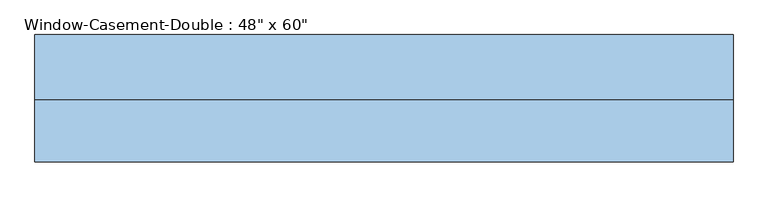
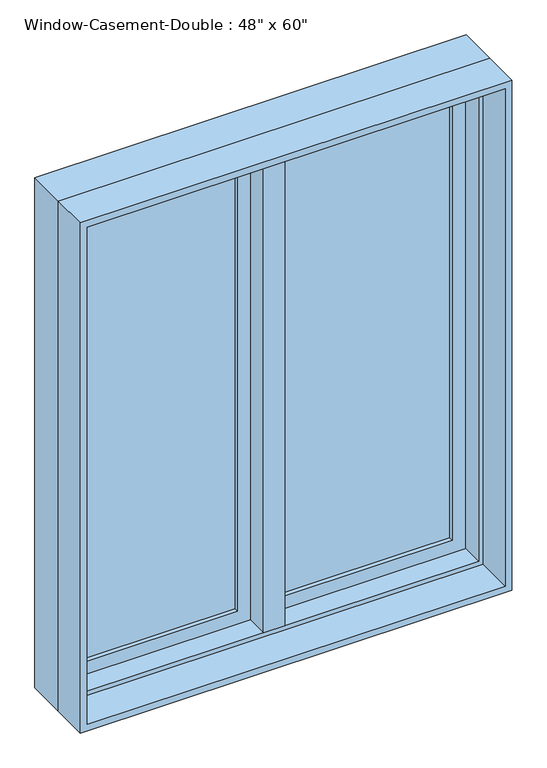
"""IFC4 building model written with IfcOpenShell, lengths in millimetres: window geometry."""

from ifc_helpers import new_model, si_unit, frame, origin, place, context, project, spatial, polyline, outline, extrude, faceted_brep, source, transform, mapped, element, save


def window_78633f8a(model_context):
    return source(origin(), model_context, "Body", "SolidModel", [
        faceted_brep([(9.525, 120.65, 2425.7), (-9.525, 120.65, 2425.7), (-9.525, 69.85, 2425.7), (9.525, 69.85, 2425.7), (9.525, 120.65, 927.1), (9.525, 69.85, 927.1), (-9.525, 69.85, 927.1), (-9.525, 120.65, 927.1), (-9.525, 69.85, 946.15), (-9.525, 69.85, 2406.65), (-30.1625, 69.85, 946.15), (-30.1625, 69.85, 2406.65), (-30.1625, 6.35, 946.15), (-30.1625, 6.35, 2406.65), (30.1625, 6.35, 946.15), (30.1625, 6.35, 2406.65), (30.1625, 69.85, 946.15), (30.1625, 69.85, 2406.65), (9.525, 69.85, 946.15), (9.525, 69.85, 2406.65)], [[[0, 1, 2, 3]], [[4, 5, 6, 7]], [[1, 0, 4, 7]], [[2, 1, 7, 6, 8, 9]], [[9, 8, 10, 11]], [[11, 10, 12, 13]], [[13, 12, 14, 15]], [[15, 14, 16, 17]], [[17, 16, 18, 19]], [[0, 3, 19, 18, 5, 4]], [[18, 8, 6, 5]], [[9, 19, 3, 2]], [[8, 18, 16, 14, 12, 10]], [[19, 9, 11, 13, 15, 17]]]),
        extrude(outline(polyline([(-66.675, 101.6), (-66.675, 95.25), (-539.75, 95.25), (-539.75, 101.6), (-66.675, 101.6)])), frame((0.0, 0.0, 984.25), z_axis=(0.0, 0.0, 1.0), x_axis=(1.0, 0.0, 0.0)), (0.0, 0.0, 1.0), 1384.3),
        extrude(outline(polyline([(-539.75, 82.55), (-539.75, 88.9), (-66.675, 88.9), (-66.675, 82.55), (-539.75, 82.55)])), frame((0.0, 0.0, 984.25), z_axis=(0.0, 0.0, 1.0), x_axis=(1.0, 0.0, 0.0)), (0.0, 0.0, 1.0), 1384.3),
        extrude(outline(polyline([(539.75, 101.6), (539.75, 95.25), (66.675, 95.25), (66.675, 101.6), (539.75, 101.6)])), frame((0.0, 0.0, 984.25), z_axis=(0.0, 0.0, 1.0), x_axis=(1.0, 0.0, 0.0)), (0.0, 0.0, 1.0), 1384.3),
        extrude(outline(polyline([(66.675, 82.55), (66.675, 88.9), (539.75, 88.9), (539.75, 82.55), (66.675, 82.55)])), frame((0.0, 0.0, 984.25), z_axis=(0.0, 0.0, 1.0), x_axis=(1.0, 0.0, 0.0)), (0.0, 0.0, 1.0), 1384.3),
        extrude(outline(polyline([(2425.7, -596.9), (927.1, -596.9), (927.1, -9.525), (2425.7, -9.525), (2425.7, -596.9)]), holes=[polyline([(2368.55, -66.675), (984.25, -66.675), (984.25, -539.75), (2368.55, -539.75), (2368.55, -66.675)])]), frame((0.0, 69.85, 0.0), z_axis=(0.0, 1.0, 0.0), x_axis=(0.0, 0.0, 1.0)), (0.0, 0.0, 1.0), 44.45),
        extrude(outline(polyline([(927.1, 596.9), (2425.7, 596.9), (2425.7, 9.525), (927.1, 9.525), (927.1, 596.9)]), holes=[polyline([(984.25, 66.675), (2368.55, 66.675), (2368.55, 539.75), (984.25, 539.75), (984.25, 66.675)])]), frame((0.0, 69.85, 0.0), z_axis=(0.0, 1.0, 0.0), x_axis=(0.0, 0.0, 1.0)), (0.0, 0.0, 1.0), 44.45),
        extrude(outline(polyline([(2438.4, -609.6), (914.4, -609.6), (914.4, 609.6), (2438.4, 609.6), (2438.4, -609.6)]), holes=[polyline([(2419.35, 590.55), (933.45, 590.55), (933.45, -590.55), (2419.35, -590.55), (2419.35, 590.55)])]), frame((0.0, -101.6, 0.0), z_axis=(0.0, 1.0, 0.0), x_axis=(0.0, 0.0, 1.0)), (0.0, 0.0, 1.0), 107.95),
        faceted_brep([(577.85, 69.85, 2406.65), (577.85, 6.35, 2406.65), (-577.85, 6.35, 2406.65), (-577.85, 69.85, 2406.65), (596.9, 120.65, 2425.7), (596.9, 69.85, 2425.7), (-596.9, 69.85, 2425.7), (-596.9, 120.65, 2425.7), (609.6, 6.35, 2438.4), (609.6, 120.65, 2438.4), (-609.6, 120.65, 2438.4), (-609.6, 6.35, 2438.4), (-577.85, 6.35, 946.15), (-577.85, 69.85, 946.15), (-596.9, 69.85, 927.1), (-596.9, 120.65, 927.1), (-609.6, 120.65, 914.4), (-609.6, 6.35, 914.4), (577.85, 6.35, 946.15), (577.85, 69.85, 946.15), (596.9, 69.85, 927.1), (596.9, 120.65, 927.1), (609.6, 120.65, 914.4), (609.6, 6.35, 914.4)], [[[0, 1, 2, 3]], [[4, 5, 6, 7]], [[8, 9, 10, 11]], [[3, 2, 12, 13]], [[7, 6, 14, 15]], [[11, 10, 16, 17]], [[13, 12, 18, 19]], [[15, 14, 20, 21]], [[17, 16, 22, 23]], [[11, 17, 23, 8], [1, 18, 12, 2]], [[19, 18, 1, 0]], [[5, 20, 14, 6], [3, 13, 19, 0]], [[21, 20, 5, 4]], [[23, 22, 9, 8]], [[9, 22, 16, 10], [7, 15, 21, 4]]]),
    ])


if __name__ == "__main__":
    model = new_model("IFC4")
    model_context = context("Model", 3, world=origin())
    ifc_project = project(units=[si_unit("LENGTHUNIT", "METRE", prefix="MILLI")], contexts=[model_context])
    site = spatial("IfcSite", under=ifc_project)
    building = spatial("IfcBuilding", under=site)
    placement = place(None, origin())
    window_shape = window_78633f8a(model_context)
    element("IfcWindow", 1, ObjectType="Window-Casement-Double : 48\" x 60\"", at=placement, inside=building, context=model_context, shape_type="MappedRepresentation", body=[
        mapped(window_shape, transform((0.0, 0.0, 0.0), x_axis=(1.0, 0.0, 0.0), y_axis=(0.0, 1.0, 0.0), z_axis=(0.0, 0.0, 1.0))),
    ])
    save(model, "model.ifc")

# Revit data of these elements
# Type "Window-Casement-Double : 48\" x 60\""
#   Type Mark = "61"
#   Fire Rating = "0.5h"
#   Assembly Code = "B2020100"
#   Analytic Construction = "Double glazing - domestic"
#   Frame Extension [instance default] = 0' - 0 1/4"
#   Window Inset [instance default] = 0' - 0"
#   Wall Thickness [instance default] = 0' - 6"
#   Interior Wall Closure [instance default] = 0' - 2 1/4"
#   Half Width = 2' - 0"
#   Visual Light Transmittance = 0.81
#   Thermal Resistance (R) = 1.8146 (h·ft²·°F)/BTU
#   Solar Heat Gain Coefficient = 0.76
#   Rough Width = 4' - 0 1/2"
#   Rough Height = 5' - 0 1/2"
#   Height = 5' - 0"
#   Heat Transfer Coefficient (U) = 0.5511 BTU/(h·ft²·°F)
#   Exterior Wall Closure [instance default] = 0' - 1 1/4"
#   Extension Jamb [instance default] = 0' - 2 1/4"
#   Default Sill Height = 3' - 0"
#   Width = 4' - 0"
#   Define Thermal Properties by = 0
#   Muntin Visibility = yes
#   Interior Trim Visibility [instance default] = yes
#   Exterior Trim Visibility [instance default] = yes
#   Extension Jamb Visibility [instance default] = yes
#   Interior Trim Material = Wood - Stained
#   Muntin Pattern = Muntin Pattern_2x2 : Muntin Pattern_2x2
#   Interior Trim = Trim-Window-Interior-Flat : Picture Frame
#   Interior Frame Material = Wood - Stained
#   Glass Panel Material = Glass
#   Exterior Trim Material = Clad - White
#   Exterior Trim = Trim-Window-Exterior-Flat : with Sill
#   Exterior Frame Material = Clad - White
#   Wall Closure = (empty or 0)
# Element 1 (IfcWindow, "Window-Casement-Double : 48\" x 60\"")
#   Wall Thickness = 0' - 8"
#   Extension Jamb = 0' - 4 1/4"
#   Materials on its faces: "Wood - Stained", "Glass", "Clad - White"
# Materials
#   "Wood - Stained": class "Wood", colour RGB 224 178 126, transparency 0, Cost = 0
#   "Glass": class "Glass", colour RGB 236 240 239, transparency 0.5, Description = "Soda Lime Glass", Cost = 0
#   "Clad - White": class "Wood", colour RGB 216 216 204, transparency 0, Cost = 0
